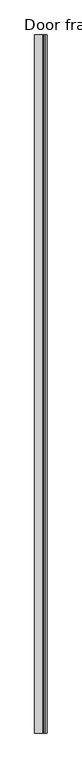
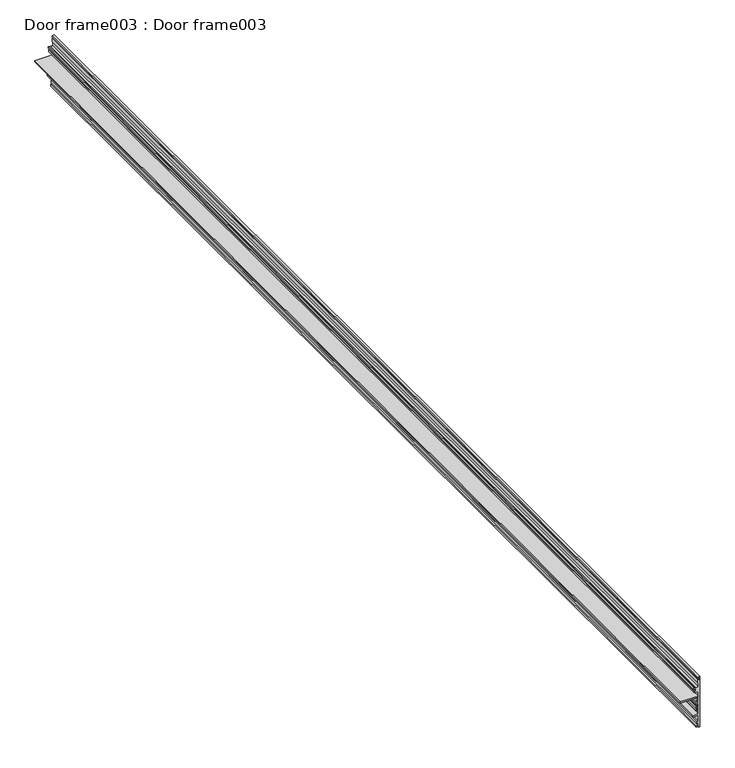
"""IFC4 building model written with IfcOpenShell, lengths in millimetres: proxy geometry, Door frame003 : Door frame003."""

from ifc_helpers import new_model, si_unit, frame, origin, place, context, project, spatial, polyline, outline, extrude, source, transform, mapped, element, save


def door_frame003_door_frame003_8b51607b(model_context):
    return source(origin(), model_context, "Body", "SweptSolid", [
        extrude(outline(polyline([(36640.7292623, 15558.7942271), (36638.6348329, 15558.7942271), (36638.6348329, 15555.2376968), (36635.0786991, 15555.2376968), (36635.0786991, 15556.6349454), (36637.237374, 15556.6349454), (36637.237374, 15558.7933141), (36629.3636227, 15558.7933141), (36629.3636227, 15556.634085), (36631.522833, 15556.634085), (36631.522833, 15555.2366262), (36627.9663742, 15555.2366262), (36627.9663742, 15558.7925325), (36625.8711226, 15558.7925325), (36625.8711226, 15556.6360862), (36624.9183358, 15554.7312296), (36623.9664094, 15556.636373), (36623.9664094, 15558.7925159), (36617.0240434, 15558.7925159), (36617.0240434, 15549.0103859), (36613.8490434, 15549.0103859), (36613.8490434, 15558.7893859), (36602.905231, 15558.7893859), (36602.905231, 15556.3015659), (36598.5961003, 15556.3015659), (36600.1211436, 15558.8008339), (36594.775583, 15558.8008339), (36595.6486981, 15555.544285), (36592.4137824, 15555.2607758), (36593.5561506, 15557.6006351), (36593.5561506, 15558.9588558), (36591.6240434, 15558.9588558), (36591.6240434, 15561.9764133), (36686.8713846, 15561.9764133), (36686.8713846, 15557.8513976), (36684.2230088, 15557.8513976), (36684.2230088, 15559.1060732), (36685.5545864, 15559.1060732), (36685.5545864, 15560.591093), (36680.6298938, 15560.591093), (36680.6298938, 15559.1060732), (36681.9249044, 15559.1060732), (36681.9249044, 15557.8513976), (36675.7714394, 15557.8513976), (36675.7714394, 15559.0526143), (36667.7720071, 15559.0526143), (36667.7720071, 15554.3561718), (36667.5392258, 15553.1571189), (36668.6824408, 15550.8176037), (36665.4474399, 15551.1001389), (36666.3193526, 15554.3561219), (36660.9960694, 15554.3561219), (36662.4395074, 15551.856014), (36658.8017047, 15551.856014), (36658.8017047, 15558.7960921), (36650.6101085, 15558.7960921), (36650.6101085, 15527.0514077), (36648.0323358, 15527.0514077), (36648.0323358, 15558.795388), (36642.634549, 15558.795388), (36642.634549, 15556.636373), (36641.6823358, 15554.7312296), (36640.7292623, 15556.6360862), (36640.7292623, 15558.7942271)])), frame((0.0, -1052.8906567, 0.0), z_axis=(0.0, 1.0, 0.0), x_axis=(0.0, 0.0, 1.0)), (0.0, 0.0, 1.0), 1999.85),
    ])


if __name__ == "__main__":
    model = new_model("IFC4")
    model_context = context("Model", 3, world=origin())
    ifc_project = project(units=[si_unit("LENGTHUNIT", "METRE", prefix="MILLI")], contexts=[model_context])
    site = spatial("IfcSite", under=ifc_project)
    building = spatial("IfcBuilding", under=site)
    placement = place(None, origin())
    door_frame003_door_frame003_shape = door_frame003_door_frame003_8b51607b(model_context)
    element("IfcBuildingElementProxy", 1, Name="Door frame003 : Door frame003", ObjectType="Door frame003 : Door frame003", at=placement, inside=building, context=model_context, shape_type="MappedRepresentation", body=[
        mapped(door_frame003_door_frame003_shape, transform((0.0, 0.0, 0.0), x_axis=(1.0, 0.0, 0.0), y_axis=(0.0, 1.0, 0.0), z_axis=(0.0, 0.0, 1.0))),
    ])
    save(model, "model.ifc")

# Revit data of these elements
# Type "Door frame003 : Door frame003"
#   NameOverride = "Door frame003"
# Element 1 (IfcBuildingElementProxy, "Door frame003 : Door frame003")
#   Materials on its faces: "FLEETWOOD SERIES T-3200 SINGLE SWING DOOR FRAME"
# Materials
#   "FLEETWOOD SERIES T-3200 SINGLE SWING DOOR FRAME": class "Unassigned", colour RGB 128 128 128, transparency 0, Cost = 0
